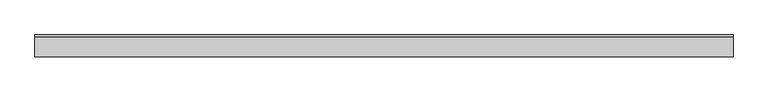
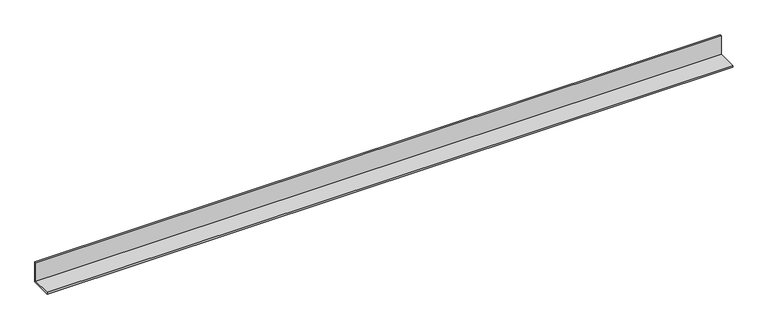
"""IFC4 building model written with IfcOpenShell, lengths in millimetres: proxy geometry, Generic Models 7:Generic Models 1:5:Generic Models 1:5 : Generic Models 7:Generic Models 1:337419:12 : Generic Models 7:Generic Models 1:5:Generic Models 1:5 : Generic Models 7:Generic Models 1:337419:311462."""

from ifc_helpers import new_model, si_unit, frame, origin, place, context, project, spatial, polyline, outline, extrude, source, transform, mapped, element, save


def generic_models_b83e92c5(model_context):
    return source(origin(), model_context, "Body", "SweptSolid", [
        extrude(outline(polyline([(-579013.3913841, 3708.4), (-579089.5913841, 3708.4), (-579089.5913841, 3714.75), (-579019.7413841, 3714.75), (-579019.7413841, 3784.6), (-579013.3913841, 3784.6), (-579013.3913841, 3708.4)])), frame((568007.8867239, 0.0, 0.0), z_axis=(1.0, 0.0, 0.0), x_axis=(0.0, 1.0, 0.0)), (0.0, 0.0, 1.0), 2444.75),
    ])


if __name__ == "__main__":
    model = new_model("IFC4")
    model_context = context("Model", 3, world=origin())
    ifc_project = project(units=[si_unit("LENGTHUNIT", "METRE", prefix="MILLI")], contexts=[model_context])
    site = spatial("IfcSite", under=ifc_project)
    building = spatial("IfcBuilding", under=site)
    placement = place(None, origin())
    generic_models_shape = generic_models_b83e92c5(model_context)
    element("IfcBuildingElementProxy", 1, Name="Generic Models 7:Generic Models 1:5:Generic Models 1:5 : Generic Models 7:Generic Models 1:337419:12 : Generic Models 7:Generic Models 1:5:Generic Models 1:5 : Generic Models 7:Generic Models 1:337419:311462", ObjectType="Generic Models 7:Generic Models 1:5:Generic Models 1:5 : Generic Models 7:Generic Models 1:337419:12 : Generic Models 7:Generic Models 1:5:Generic Models 1:5 : Generic Models 7:Generic Models 1:337419:311462", at=placement, inside=building, context=model_context, shape_type="MappedRepresentation", body=[
        mapped(generic_models_shape, transform((0.0, 0.0, 0.0), x_axis=(1.0, 0.0, 0.0), y_axis=(0.0, 1.0, 0.0), z_axis=(0.0, 0.0, 1.0))),
    ])
    save(model, "model.ifc")

# Revit data of these elements
# Type "Generic Models 7:Generic Models 1:5:Generic Models 1:5 : Generic Models 7:Generic Models 1:337419:12 : Generic Models 7:Generic Models 1:5:Generic Models 1:5 : Generic Models 7:Generic Models 1:337419:311462"
#   NameOverride = "Generic Models 7:Generic Models 1:5:Generic Models 1:5 : Generic Models 7:Generic Models 1:337419:311462"
#   ObjectTypeOverride = "Generic Models 1:5 : Generic Models 7:Generic Models 1:337419"
#   Reference = "Generic Models 1"
#   Tag = "311462"
# Element 1 (IfcBuildingElementProxy, "Generic Models 7:Generic Models 1:5:Generic Models 1:5 : Generic Models 7:Generic Models 1:337419:12 : Generic Models 7:Generic Models 1:5:Generic Models 1:5 : Generic Models 7:Generic Models 1:337419:311462")
#   Materials on its faces: "STRUCTURAL STEEL - SEE STRUCT. DWGS"
# Materials
#   "STRUCTURAL STEEL - SEE STRUCT. DWGS": class "Metal", colour RGB 189 187 185, transparency 0, Description = "Structural steel 50ksi", Cost = 0
